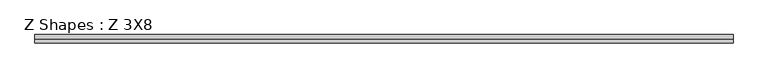
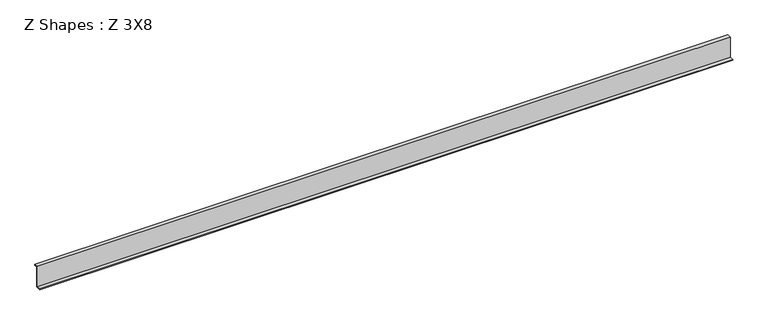
"""IFC4 building model written with IfcOpenShell, lengths in millimetres: beam geometry, Z Shapes : Z 3X8."""

from ifc_helpers import new_model, si_unit, frame, origin, place, context, project, spatial, polyline, outline, extrude, source, transform, mapped, element, save


def z_shapes_z_3x8_52d35dee(model_context):
    return source(origin(), model_context, "Body", "SweptSolid", [
        extrude(outline(polyline([(57.2805719, 92.452825), (27.1991352, 92.452825), (27.1991352, -98.809175), (-18.9194281, -98.809175), (-18.9194281, -92.459175), (19.1805719, -92.459175), (19.1805719, 102.104825), (57.2805719, 102.104825), (57.2805719, 92.452825)])), frame((-3168.65, 0.0, 0.0), z_axis=(1.0, 0.0, 0.0), x_axis=(0.0, 1.0, 0.0)), (0.0, 0.0, 1.0), 6337.3),
    ])


if __name__ == "__main__":
    model = new_model("IFC4")
    model_context = context("Model", 3, world=origin())
    ifc_project = project(units=[si_unit("LENGTHUNIT", "METRE", prefix="MILLI")], contexts=[model_context])
    site = spatial("IfcSite", under=ifc_project)
    building = spatial("IfcBuilding", under=site)
    placement = place(None, origin())
    z_shapes_z_3x8_shape = z_shapes_z_3x8_52d35dee(model_context)
    element("IfcBeam", 1, ObjectType="Z Shapes : Z 3X8", at=placement, inside=building, context=model_context, shape_type="MappedRepresentation", body=[
        mapped(z_shapes_z_3x8_shape, transform((0.0, 0.0, 0.0), x_axis=(1.0, 0.0, 0.0), y_axis=(0.0, 1.0, 0.0), z_axis=(0.0, 0.0, 1.0))),
    ])
    save(model, "model.ifc")

# Revit data of these elements
# Type "Z Shapes : Z 3X8"
#   Section Name Key = "W12x26"
#   Assembly Code = "B10"
#   Width = 76.2 mm
#   Web Thickness = 5.842 mm
#   Web Fillet = 7.62 mm
#   Warping Constant = 163001.3 cm⁶
#   Torsional Moment of Inertia = 12.4869 cm⁴
#   Section Area = 7.65 in²
#   Plastic Modulus weak axis = 0.00472801 (stored number, unit not read)
#   Plastic Modulus strong axis = 0.0215278 (stored number, unit not read)
#   Perimeter = 15.0571 m²/m
#   Nominal Weight = 379.441 N/m
#   Moment of Inertia weak axis = 720.08 cm⁴
#   Moment of Inertia strong axis = 8491.12 cm⁴
#   Height = 184.912 mm
#   Flange Thickness = 9.652 mm
#   Elastic Modulus weak axis = 0.00309028 (stored number, unit not read)
#   Elastic Modulus strong axis = 0.0193287 (stored number, unit not read)
#   Centroid Vertical = 92.456 mm
#   Centroid Horizontal = 38.1 mm
#   Length [instance default] = 5' - 0"
#   Structural Material [instance default] = Steel ASTM A992
#   Principal Axes Angle = 0
# Element 1 (IfcBeam, "Z Shapes : Z 3X8")
#   Structural Material = accent 2
#   Materials on its faces: "accent 2"
# Materials
#   "Steel ASTM A992": class "Metal", colour RGB 189 187 185, transparency 0, Description = "Structural steel 50ksi", Cost = 0
#   "accent 2": class "Wood", colour RGB 80 80 80, transparency 0, Description = "Wood framing, thermal airspace", Cost = 0
